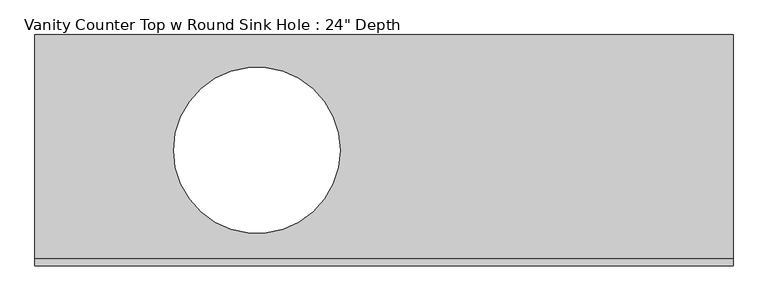
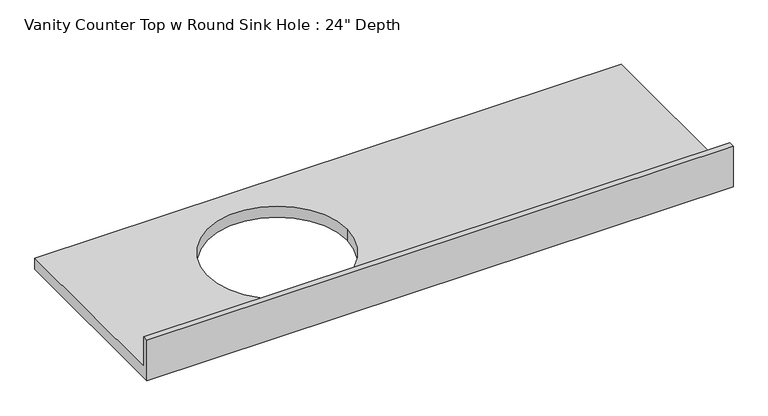
"""IFC4 building model written with IfcOpenShell, lengths in millimetres: furniture geometry."""

import ifcopenshell
import ifcopenshell.guid

model = None  # the IFC model being written
_history = None  # IfcOwnerHistory: only IFC2X3 demands one
_inside = {}  # id of a spatial element -> (the spatial element, [elements in it])
_under = {}  # id of a project, library or spatial element -> (it, [spatial elements below it])
_declared = {}  # id of a project -> (the project, [libraries it declares])
_typed = {}  # id of a type object -> (the type object, [elements of that type])
_made_of = {}  # id of a material, layer set ... -> (it, [elements and type objects made of it])


def new_model(schema):
    """Start an empty IFC model of exactly this schema.

    Asked for "IFC4X3", IfcOpenShell would pick the latest addendum, in which some entities
    have other attributes; the version numbers below select the first issue.
    IFC2X3 requires an IfcOwnerHistory on every rooted entity: one is made here for all.
    """
    global model, _history
    if schema == "IFC4X3":
        model = ifcopenshell.file(schema_version=(4, 3, 0, 0))
    else:
        model = ifcopenshell.file(schema=schema)
    _inside.clear()
    _under.clear()
    _declared.clear()
    _typed.clear()
    _made_of.clear()
    _history = None
    if model.schema == "IFC2X3":
        org = make("IfcOrganization", Name="unknown")
        user = make(
            "IfcPersonAndOrganization",
            ThePerson=make("IfcPerson", FamilyName="unknown"),
            TheOrganization=org,
        )
        app = make(
            "IfcApplication",
            ApplicationDeveloper=org,
            Version="unknown",
            ApplicationFullName="unknown",
            ApplicationIdentifier="unknown",
        )
        _history = make(
            "IfcOwnerHistory",
            OwningUser=user,
            OwningApplication=app,
            ChangeAction="ADDED",
            CreationDate=0,
        )
    return model


def make(cls, **values):
    """One entity of the class cls with the attributes given. An attribute that is None is left unset."""
    return model.create_entity(
        cls, **{name: value for name, value in values.items() if value is not None}
    )


def rooted(cls, **values):
    """An entity with a GlobalId (a new one), such as an element, a storey or a relation."""
    return make(cls, GlobalId=ifcopenshell.guid.new(), OwnerHistory=_history, **values)


def si_unit(unit_type, name, prefix=None):
    """IfcSIUnit, for example si_unit("LENGTHUNIT", "METRE", prefix="MILLI")."""
    return make("IfcSIUnit", UnitType=unit_type, Prefix=prefix, Name=name)


def assignment(units):
    """IfcUnitAssignment: the units of a project."""
    return None if units is None else make("IfcUnitAssignment", Units=units)


def point(xyz):
    """IfcCartesianPoint."""
    return None if xyz is None else make("IfcCartesianPoint", Coordinates=xyz)


def direction(xyz):
    """IfcDirection."""
    return None if xyz is None else make("IfcDirection", DirectionRatios=xyz)


def frame(location, z_axis=None, x_axis=None):
    """IfcAxis2Placement3D, a coordinate frame: its origin and axes. An axis left out is left unset."""
    return make(
        "IfcAxis2Placement3D",
        Location=point(location),
        Axis=direction(z_axis),
        RefDirection=direction(x_axis),
    )


def origin():
    """The frame at (0, 0, 0) with its axes left unset."""
    return frame((0.0, 0.0, 0.0))


def place(relative_to, where):
    """IfcLocalPlacement: puts the frame where relative to a parent placement (None: the world)."""
    return make(
        "IfcLocalPlacement", PlacementRelTo=relative_to, RelativePlacement=where
    )


def context(
    kind, dimensions, precision=None, world=None, true_north=None, identifier=None
):
    """IfcGeometricRepresentationContext, for example the 3D "Model" context."""
    return make(
        "IfcGeometricRepresentationContext",
        ContextIdentifier=identifier,
        ContextType=kind,
        CoordinateSpaceDimension=dimensions,
        Precision=precision,
        WorldCoordinateSystem=world,
        TrueNorth=true_north,
    )


def project(units=None, contexts=None):
    """IfcProject with its units and contexts."""
    return rooted(
        "IfcProject",
        Name="project",
        RepresentationContexts=contexts,
        UnitsInContext=assignment(units),
    )


def spatial(cls, under=None, at=None, **own):
    """A site, building, storey or space (cls), placed at a placement, below another one or the project."""
    s = rooted(cls, ObjectPlacement=at, **own)
    if under is not None:
        _under.setdefault(under.id(), (under, []))[1].append(s)
    return s


def polyline(points):
    """IfcPolyline through the points."""
    return make("IfcPolyline", Points=[point(p) for p in points])


def circle_curve(where, radius):
    """IfcCircle in the frame where."""
    return make("IfcCircle", Position=where, Radius=radius)


def shape(context_of_items, identifier, shape_type, items):
    """IfcShapeRepresentation: the items that make up one representation, for example the "Body"."""
    return make(
        "IfcShapeRepresentation",
        ContextOfItems=context_of_items,
        RepresentationIdentifier=identifier,
        RepresentationType=shape_type,
        Items=items,
    )


def source(mapping_origin, context_of_items, identifier, shape_type, items):
    """IfcRepresentationMap: a shape defined once, which mapped items show again and again."""
    return make(
        "IfcRepresentationMap",
        MappingOrigin=mapping_origin,
        MappedRepresentation=shape(context_of_items, identifier, shape_type, items),
    )


def transform(
    local_origin,
    x_axis=None,
    y_axis=None,
    z_axis=None,
    scale=None,
    scale2=None,
    scale3=None,
    uniform=True,
):
    """IfcCartesianTransformationOperator3D, or its non-uniform kind. x_axis, y_axis, z_axis: its Axis1, 2, 3."""
    if uniform:
        return make(
            "IfcCartesianTransformationOperator3D",
            Axis1=direction(x_axis),
            Axis2=direction(y_axis),
            LocalOrigin=point(local_origin),
            Scale=scale,
            Axis3=direction(z_axis),
        )
    return make(
        "IfcCartesianTransformationOperator3DnonUniform",
        Axis1=direction(x_axis),
        Axis2=direction(y_axis),
        LocalOrigin=point(local_origin),
        Scale=scale,
        Axis3=direction(z_axis),
        Scale2=scale2,
        Scale3=scale3,
    )


def mapped(mapping_source, mapping_target):
    """IfcMappedItem: shows the shape of a source again, moved by a transform."""
    return make(
        "IfcMappedItem", MappingSource=mapping_source, MappingTarget=mapping_target
    )


def made_of(thing, what):
    """Note that an element or type object is made of a material, layer set ...; save() writes the relation."""
    if what is not None:
        _made_of.setdefault(what.id(), (what, []))[1].append(thing)
    return thing


def element(
    cls,
    number,
    at=None,
    inside=None,
    cuts=None,
    type_object=None,
    material=None,
    context=None,
    identifier="Body",
    shape_type=None,
    held_by="IfcProductDefinitionShape",
    body=None,
    shapes=None,
    **own,
):
    """One element of the class cls, such as IfcWall. Its Tag is "e" and its number.

    at: its placement. inside: the storey or other place that contains it. cuts: it is an
    opening in that element (IfcRelVoidsElement). A single representation is given by context,
    identifier, shape_type and body (its items); several are given by shapes. held_by: the class
    of the entity that holds the representations. save() writes the other relations.
    """
    e = rooted(cls, Tag="e%d" % number, ObjectPlacement=at, **own)
    if body is not None:
        shapes = [shape(context, identifier, shape_type, body)]
    if shapes is not None:
        e.Representation = make(held_by, Representations=shapes)
    if inside is not None:
        _inside.setdefault(inside.id(), (inside, []))[1].append(e)
    if cuts is not None:
        rooted(
            "IfcRelVoidsElement", RelatingBuildingElement=cuts, RelatedOpeningElement=e
        )
    if type_object is not None:
        _typed.setdefault(type_object.id(), (type_object, []))[1].append(e)
    return made_of(e, material)


def aggregate(whole, parts):
    """IfcRelAggregates: a whole, such as a stair, and the parts it consists of."""
    return rooted("IfcRelAggregates", RelatingObject=whole, RelatedObjects=parts)


def save(model, path):
    """Write the relations noted so far, then the file.

    IfcRelAggregates (storeys below a building ...), IfcRelContainedInSpatialStructure (elements
    in a storey), IfcRelDefinesByType, IfcRelAssociatesMaterial and IfcRelDeclares: one each for
    every whole, place, type object, material and project.
    """
    for whole, parts in _under.values():
        aggregate(whole, parts)
    for where, things in _inside.values():
        rooted(
            "IfcRelContainedInSpatialStructure",
            RelatedElements=things,
            RelatingStructure=where,
        )
    for kind, things in _typed.values():
        rooted("IfcRelDefinesByType", RelatedObjects=things, RelatingType=kind)
    for what, things in _made_of.values():
        rooted("IfcRelAssociatesMaterial", RelatedObjects=things, RelatingMaterial=what)
    for by, libraries in _declared.values():
        rooted("IfcRelDeclares", RelatingContext=by, RelatedDefinitions=libraries)
    model.write(path)


def plane_surface(at):
    """IfcPlane: the flat surface through the origin of the frame at, square to its z axis."""
    return make("IfcPlane", Position=at)


def revolved_surface(curve, axis_point, axis_direction):
    """IfcSurfaceOfRevolution: the curve turned about the line through axis_point along axis_direction."""
    return make(
        "IfcSurfaceOfRevolution",
        SweptCurve=make("IfcArbitraryOpenProfileDef", ProfileType="CURVE", Curve=curve),
        AxisPosition=make("IfcAxis1Placement", Location=point(axis_point), Axis=direction(axis_direction)),
    )


def advanced_brep(points, edges, surfaces, faces):
    """IfcAdvancedBrep: a solid bounded by faces that lie on surfaces and meet in shared edges.

    An edge is (start, end): straight between two places in points (the first is 0);
    or (start, end, curve); or (start, end, curve, False) where it runs against its curve.
    A face is (place in surfaces, loops), or (place, loops, False) where it looks against
    its surface's normal. A loop lists edges by number (the first is 1), with a minus sign
    where the edge is run from its end to its start. The first loop is the outer one.
    """
    corners = [point(p) for p in points]
    vertices = [make("IfcVertexPoint", VertexGeometry=c) for c in corners]
    made = []
    for start, end, *more in edges:
        made.append(
            make(
                "IfcEdgeCurve",
                EdgeStart=vertices[start],
                EdgeEnd=vertices[end],
                EdgeGeometry=more[0] if more else make("IfcPolyline", Points=[corners[start], corners[end]]),
                SameSense=more[1] if len(more) > 1 else True,
            )
        )
    hull = []
    for where, loops, *sense in faces:
        bounds = []
        for j, loop in enumerate(loops):
            ring = [make("IfcOrientedEdge", EdgeElement=made[abs(k) - 1], Orientation=k > 0) for k in loop]
            bounds.append(
                make(
                    "IfcFaceOuterBound" if j == 0 else "IfcFaceBound",
                    Bound=make("IfcEdgeLoop", EdgeList=ring),
                    Orientation=True,
                )
            )
        hull.append(make("IfcAdvancedFace", Bounds=bounds, FaceSurface=surfaces[where], SameSense=sense[0] if sense else True))
    return make("IfcAdvancedBrep", Outer=make("IfcClosedShell", CfsFaces=hull))


def furniture_cfdb0dcc(model_context):
    return source(origin(), model_context, "Body", "AdvancedBrep", [
        advanced_brep(
        [(-1327.4622951, 635.0, 787.4), (-1327.4622951, 19.05, 787.4), (590.2377049, 19.05, 787.4), (590.2377049, 635.0, 787.4), (-489.2622951, 317.5, 787.4), (-946.4622951, 317.5, 787.4), (590.2377049, 0.0, 749.3), (-1327.4622951, 0.0, 749.3), (-1327.4622951, 635.0, 749.3), (590.2377049, 635.0, 749.3), (-946.4622951, 317.5, 749.3), (-489.2622951, 317.5, 749.3), (590.2377049, 0.0, 889.0), (-1327.4622951, 0.0, 889.0), (-1327.4622951, 19.05, 889.0), (590.2377049, 19.05, 889.0)],
        [
            (0, 1),
            (1, 2),
            (2, 3),
            (3, 0),
            (4, 5, circle_curve(frame((-717.8622951, 317.5, 787.4), z_axis=(0.0, 0.0, -1.0), x_axis=(1.0, 0.0, 0.0)), 228.6)),
            (5, 4, circle_curve(frame((-717.8622951, 317.5, 787.4), z_axis=(0.0, 0.0, -1.0), x_axis=(1.0, 0.0, 0.0)), 228.6)),
            (6, 7),
            (7, 8),
            (8, 9),
            (9, 6),
            (10, 11, circle_curve(frame((-717.8622951, 317.5, 749.3), z_axis=(0.0, 0.0, 1.0), x_axis=(1.0, 0.0, 0.0)), 228.6)),
            (11, 10, circle_curve(frame((-717.8622951, 317.5, 749.3), z_axis=(0.0, 0.0, 1.0), x_axis=(1.0, 0.0, 0.0)), 228.6)),
            (6, 12),
            (12, 13),
            (13, 7),
            (13, 14),
            (14, 1),
            (0, 8),
            (3, 9),
            (2, 15),
            (15, 12),
            (15, 14),
            (5, 10),
            (11, 4),
        ],
        [
            plane_surface(frame((-1327.4622951, 0.0, 787.4), z_axis=(0.0, 0.0, 1.0), x_axis=(-1.0, 0.0, 0.0))),
            plane_surface(frame((-1327.4622951, 0.0, 749.3), z_axis=(0.0, 0.0, -1.0), x_axis=(1.0, 0.0, 0.0))),
            plane_surface(frame((590.2377049, 0.0, 787.4), z_axis=(0.0, -1.0, 0.0), x_axis=(0.0, 0.0, -1.0))),
            plane_surface(frame((-1327.4622951, 0.0, 787.4), z_axis=(-1.0, 0.0, 0.0), x_axis=(0.0, 0.0, -1.0))),
            plane_surface(frame((-1327.4622951, 635.0, 787.4), z_axis=(0.0, 1.0, 0.0), x_axis=(0.0, 0.0, -1.0))),
            plane_surface(frame((590.2377049, 635.0, 787.4), z_axis=(1.0, 0.0, 0.0), x_axis=(0.0, 0.0, -1.0))),
            plane_surface(frame((-1327.4622951, 0.0, 889.0), z_axis=(0.0, 0.0, 1.0), x_axis=(0.0, 1.0, 0.0))),
            plane_surface(frame((-1327.4622951, 19.05, 889.0), z_axis=(0.0, 1.0, 0.0), x_axis=(0.0, 0.0, -1.0))),
            revolved_surface(polyline([(-489.26229509999996, 317.5, 787.4), (-489.26229509999996, 317.5, 749.3)]), (-717.8622951, 317.5, 749.3), (0.0, 0.0, 1.0)),
        ],
        [
            (0, [[1, 2, 3, 4], [5, 6]]),
            (1, [[7, 8, 9, 10], [11, 12]]),
            (2, [[13, 14, 15, -7]]),
            (3, [[-15, 16, 17, -1, 18, -8]]),
            (4, [[19, -9, -18, -4]]),
            (5, [[-19, -3, 20, 21, -13, -10]]),
            (6, [[-14, -21, 22, -16]]),
            (7, [[-20, -2, -17, -22]]),
            (8, [[-6, 23, -12, 24]]),
            (8, [[-11, -23, -5, -24]]),
        ],
    ),
    ])


if __name__ == "__main__":
    model = new_model("IFC4")
    model_context = context("Model", 3, world=origin())
    ifc_project = project(units=[si_unit("LENGTHUNIT", "METRE", prefix="MILLI")], contexts=[model_context])
    site = spatial("IfcSite", under=ifc_project)
    building = spatial("IfcBuilding", under=site)
    placement = place(None, origin())
    furniture_shape = furniture_cfdb0dcc(model_context)
    element("IfcFurniture", 1, ObjectType="Vanity Counter Top w Round Sink Hole : 24\" Depth", at=placement, inside=building, context=model_context, shape_type="MappedRepresentation", body=[
        mapped(furniture_shape, transform((0.0, 0.0, 0.0), x_axis=(1.0, 0.0, 0.0), y_axis=(0.0, 1.0, 0.0), z_axis=(0.0, 0.0, 1.0))),
    ])
    save(model, "model.ifc")

# Revit data of these elements
# Type "Vanity Counter Top w Round Sink Hole : 24\" Depth"
#   Assembly Code = "C1030400"
#   Counter Thickness = 0' - 1 1/2"
#   Depth = 2' - 1"
#   Height = 2' - 7"
#   Length [instance default] = 4' - 0"
#   Sink Location [instance default] = 2' - 0"
#   Sink Location To Wall [instance default] = 0' - 4"
#   Sink Opening Width [instance default] = 1' - 5"
#   Counter Top Material = Laminate, Blue, Matte
#   Default Elevation = 0
# Element 1 (IfcFurniture, "Vanity Counter Top w Round Sink Hole : 24\" Depth")
#   Length = 6' - 3 1/2"
#   Materials on its faces: "Laminate, Blue, Matte"
# Materials
#   "Laminate, Blue, Matte": class "Plastic", colour RGB 85 101 155, transparency 0, Description = "Plastic Laminate - Blue, Matte", Cost = 0
